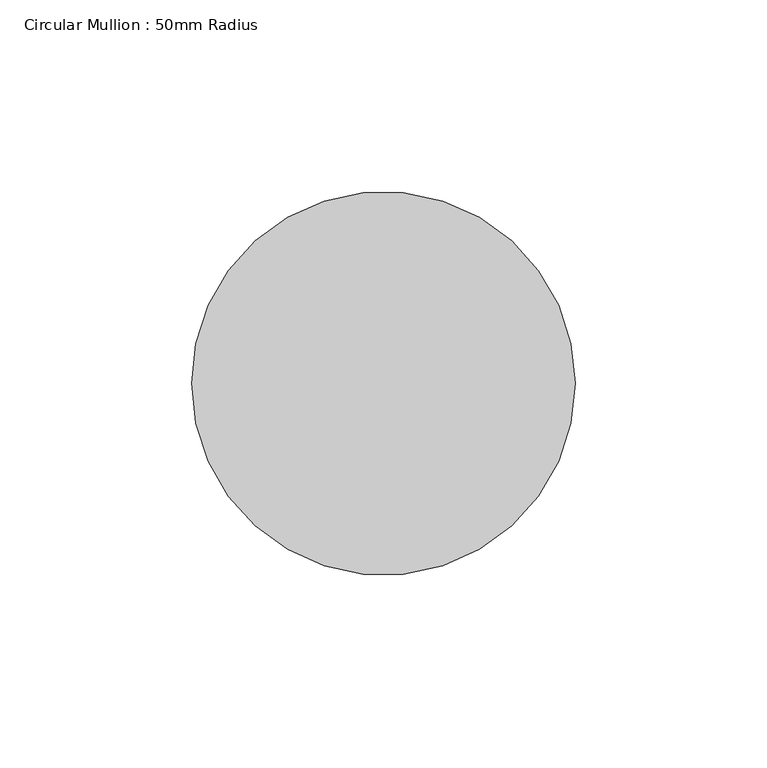
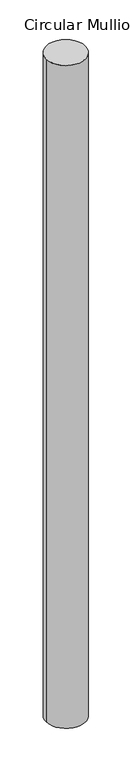
"""IFC4 building model written with IfcOpenShell, lengths in millimetres: member geometry, Circular Mullion : 50mm Radius."""

import ifcopenshell
import ifcopenshell.guid

model = None  # the IFC model being written
_history = None  # IfcOwnerHistory: only IFC2X3 demands one
_inside = {}  # id of a spatial element -> (the spatial element, [elements in it])
_under = {}  # id of a project, library or spatial element -> (it, [spatial elements below it])
_declared = {}  # id of a project -> (the project, [libraries it declares])
_typed = {}  # id of a type object -> (the type object, [elements of that type])
_made_of = {}  # id of a material, layer set ... -> (it, [elements and type objects made of it])


def new_model(schema):
    """Start an empty IFC model of exactly this schema.

    Asked for "IFC4X3", IfcOpenShell would pick the latest addendum, in which some entities
    have other attributes; the version numbers below select the first issue.
    IFC2X3 requires an IfcOwnerHistory on every rooted entity: one is made here for all.
    """
    global model, _history
    if schema == "IFC4X3":
        model = ifcopenshell.file(schema_version=(4, 3, 0, 0))
    else:
        model = ifcopenshell.file(schema=schema)
    _inside.clear()
    _under.clear()
    _declared.clear()
    _typed.clear()
    _made_of.clear()
    _history = None
    if model.schema == "IFC2X3":
        org = make("IfcOrganization", Name="unknown")
        user = make(
            "IfcPersonAndOrganization",
            ThePerson=make("IfcPerson", FamilyName="unknown"),
            TheOrganization=org,
        )
        app = make(
            "IfcApplication",
            ApplicationDeveloper=org,
            Version="unknown",
            ApplicationFullName="unknown",
            ApplicationIdentifier="unknown",
        )
        _history = make(
            "IfcOwnerHistory",
            OwningUser=user,
            OwningApplication=app,
            ChangeAction="ADDED",
            CreationDate=0,
        )
    return model


def make(cls, **values):
    """One entity of the class cls with the attributes given. An attribute that is None is left unset."""
    return model.create_entity(
        cls, **{name: value for name, value in values.items() if value is not None}
    )


def rooted(cls, **values):
    """An entity with a GlobalId (a new one), such as an element, a storey or a relation."""
    return make(cls, GlobalId=ifcopenshell.guid.new(), OwnerHistory=_history, **values)


def si_unit(unit_type, name, prefix=None):
    """IfcSIUnit, for example si_unit("LENGTHUNIT", "METRE", prefix="MILLI")."""
    return make("IfcSIUnit", UnitType=unit_type, Prefix=prefix, Name=name)


def assignment(units):
    """IfcUnitAssignment: the units of a project."""
    return None if units is None else make("IfcUnitAssignment", Units=units)


def point(xyz):
    """IfcCartesianPoint."""
    return None if xyz is None else make("IfcCartesianPoint", Coordinates=xyz)


def direction(xyz):
    """IfcDirection."""
    return None if xyz is None else make("IfcDirection", DirectionRatios=xyz)


def frame(location, z_axis=None, x_axis=None):
    """IfcAxis2Placement3D, a coordinate frame: its origin and axes. An axis left out is left unset."""
    return make(
        "IfcAxis2Placement3D",
        Location=point(location),
        Axis=direction(z_axis),
        RefDirection=direction(x_axis),
    )


def frame_2d(location, x_axis=None):
    """IfcAxis2Placement2D, a coordinate frame in the plane: its origin and x axis."""
    return make(
        "IfcAxis2Placement2D", Location=point(location), RefDirection=direction(x_axis)
    )


def origin():
    """The frame at (0, 0, 0) with its axes left unset."""
    return frame((0.0, 0.0, 0.0))


def origin_2d():
    """The frame at (0, 0) in the plane with its x axis left unset."""
    return frame_2d((0.0, 0.0))


def place(relative_to, where):
    """IfcLocalPlacement: puts the frame where relative to a parent placement (None: the world)."""
    return make(
        "IfcLocalPlacement", PlacementRelTo=relative_to, RelativePlacement=where
    )


def context(
    kind, dimensions, precision=None, world=None, true_north=None, identifier=None
):
    """IfcGeometricRepresentationContext, for example the 3D "Model" context."""
    return make(
        "IfcGeometricRepresentationContext",
        ContextIdentifier=identifier,
        ContextType=kind,
        CoordinateSpaceDimension=dimensions,
        Precision=precision,
        WorldCoordinateSystem=world,
        TrueNorth=true_north,
    )


def project(units=None, contexts=None):
    """IfcProject with its units and contexts."""
    return rooted(
        "IfcProject",
        Name="project",
        RepresentationContexts=contexts,
        UnitsInContext=assignment(units),
    )


def spatial(cls, under=None, at=None, **own):
    """A site, building, storey or space (cls), placed at a placement, below another one or the project."""
    s = rooted(cls, ObjectPlacement=at, **own)
    if under is not None:
        _under.setdefault(under.id(), (under, []))[1].append(s)
    return s


def circle_curve(where, radius):
    """IfcCircle in the frame where."""
    return make("IfcCircle", Position=where, Radius=radius)


def trimmed(basis, trim1, trim2, sense, master):
    """IfcTrimmedCurve: the piece of a basis curve between two trims."""
    return make(
        "IfcTrimmedCurve",
        BasisCurve=basis,
        Trim1=trim1,
        Trim2=trim2,
        SenseAgreement=sense,
        MasterRepresentation=master,
    )


def segment(curve, same_sense, transition):
    """IfcCompositeCurveSegment."""
    return make(
        "IfcCompositeCurveSegment",
        Transition=transition,
        SameSense=same_sense,
        ParentCurve=curve,
    )


def composite_curve(segments, self_intersect=None):
    """IfcCompositeCurve: segments joined end to end."""
    return make("IfcCompositeCurve", Segments=segments, SelfIntersect=self_intersect)


def outline(outer, holes=None, kind="AREA"):
    """IfcArbitraryClosedProfileDef: a profile drawn as a closed curve; with holes, ...WithVoids."""
    if holes is None:
        return make("IfcArbitraryClosedProfileDef", ProfileType=kind, OuterCurve=outer)
    return make(
        "IfcArbitraryProfileDefWithVoids",
        ProfileType=kind,
        OuterCurve=outer,
        InnerCurves=holes,
    )


def extrude(swept, where, along, depth):
    """IfcExtrudedAreaSolid: the profile swept, set in the frame where, extruded along a direction by depth."""
    return make(
        "IfcExtrudedAreaSolid",
        SweptArea=swept,
        Position=where,
        ExtrudedDirection=direction(along),
        Depth=depth,
    )


def shape(context_of_items, identifier, shape_type, items):
    """IfcShapeRepresentation: the items that make up one representation, for example the "Body"."""
    return make(
        "IfcShapeRepresentation",
        ContextOfItems=context_of_items,
        RepresentationIdentifier=identifier,
        RepresentationType=shape_type,
        Items=items,
    )


def source(mapping_origin, context_of_items, identifier, shape_type, items):
    """IfcRepresentationMap: a shape defined once, which mapped items show again and again."""
    return make(
        "IfcRepresentationMap",
        MappingOrigin=mapping_origin,
        MappedRepresentation=shape(context_of_items, identifier, shape_type, items),
    )


def transform(
    local_origin,
    x_axis=None,
    y_axis=None,
    z_axis=None,
    scale=None,
    scale2=None,
    scale3=None,
    uniform=True,
):
    """IfcCartesianTransformationOperator3D, or its non-uniform kind. x_axis, y_axis, z_axis: its Axis1, 2, 3."""
    if uniform:
        return make(
            "IfcCartesianTransformationOperator3D",
            Axis1=direction(x_axis),
            Axis2=direction(y_axis),
            LocalOrigin=point(local_origin),
            Scale=scale,
            Axis3=direction(z_axis),
        )
    return make(
        "IfcCartesianTransformationOperator3DnonUniform",
        Axis1=direction(x_axis),
        Axis2=direction(y_axis),
        LocalOrigin=point(local_origin),
        Scale=scale,
        Axis3=direction(z_axis),
        Scale2=scale2,
        Scale3=scale3,
    )


def mapped(mapping_source, mapping_target):
    """IfcMappedItem: shows the shape of a source again, moved by a transform."""
    return make(
        "IfcMappedItem", MappingSource=mapping_source, MappingTarget=mapping_target
    )


def made_of(thing, what):
    """Note that an element or type object is made of a material, layer set ...; save() writes the relation."""
    if what is not None:
        _made_of.setdefault(what.id(), (what, []))[1].append(thing)
    return thing


def element(
    cls,
    number,
    at=None,
    inside=None,
    cuts=None,
    type_object=None,
    material=None,
    context=None,
    identifier="Body",
    shape_type=None,
    held_by="IfcProductDefinitionShape",
    body=None,
    shapes=None,
    **own,
):
    """One element of the class cls, such as IfcWall. Its Tag is "e" and its number.

    at: its placement. inside: the storey or other place that contains it. cuts: it is an
    opening in that element (IfcRelVoidsElement). A single representation is given by context,
    identifier, shape_type and body (its items); several are given by shapes. held_by: the class
    of the entity that holds the representations. save() writes the other relations.
    """
    e = rooted(cls, Tag="e%d" % number, ObjectPlacement=at, **own)
    if body is not None:
        shapes = [shape(context, identifier, shape_type, body)]
    if shapes is not None:
        e.Representation = make(held_by, Representations=shapes)
    if inside is not None:
        _inside.setdefault(inside.id(), (inside, []))[1].append(e)
    if cuts is not None:
        rooted(
            "IfcRelVoidsElement", RelatingBuildingElement=cuts, RelatedOpeningElement=e
        )
    if type_object is not None:
        _typed.setdefault(type_object.id(), (type_object, []))[1].append(e)
    return made_of(e, material)


def aggregate(whole, parts):
    """IfcRelAggregates: a whole, such as a stair, and the parts it consists of."""
    return rooted("IfcRelAggregates", RelatingObject=whole, RelatedObjects=parts)


def save(model, path):
    """Write the relations noted so far, then the file.

    IfcRelAggregates (storeys below a building ...), IfcRelContainedInSpatialStructure (elements
    in a storey), IfcRelDefinesByType, IfcRelAssociatesMaterial and IfcRelDeclares: one each for
    every whole, place, type object, material and project.
    """
    for whole, parts in _under.values():
        aggregate(whole, parts)
    for where, things in _inside.values():
        rooted(
            "IfcRelContainedInSpatialStructure",
            RelatedElements=things,
            RelatingStructure=where,
        )
    for kind, things in _typed.values():
        rooted("IfcRelDefinesByType", RelatedObjects=things, RelatingType=kind)
    for what, things in _made_of.values():
        rooted("IfcRelAssociatesMaterial", RelatedObjects=things, RelatingMaterial=what)
    for by, libraries in _declared.values():
        rooted("IfcRelDeclares", RelatingContext=by, RelatedDefinitions=libraries)
    model.write(path)


def circular_mullion_50mm_radius_0641689d(model_context):
    return source(origin(), model_context, "Body", "SweptSolid", [
        extrude(outline(composite_curve([segment(trimmed(circle_curve(origin_2d(), 50.0), [point((50.0, 0.0))], [point((-50.0, 0.0))], False, "CARTESIAN"), True, "CONTINUOUS"), segment(trimmed(circle_curve(origin_2d(), 50.0), [point((-50.0, 0.0))], [point((50.0, 0.0))], False, "CARTESIAN"), True, "CONTINUOUS")], self_intersect=False)), frame((0.0, 0.0, -1791.6410056), z_axis=(0.0, 0.0, 1.0), x_axis=(1.0, 0.0, 0.0)), (0.0, 0.0, 1.0), 1791.6410056),
    ])


if __name__ == "__main__":
    model = new_model("IFC4")
    model_context = context("Model", 3, world=origin())
    ifc_project = project(units=[si_unit("LENGTHUNIT", "METRE", prefix="MILLI")], contexts=[model_context])
    site = spatial("IfcSite", under=ifc_project)
    building = spatial("IfcBuilding", under=site)
    placement = place(None, origin())
    circular_mullion_50mm_radius_shape = circular_mullion_50mm_radius_0641689d(model_context)
    element("IfcMember", 1, ObjectType="Circular Mullion : 50mm Radius", at=placement, inside=building, context=model_context, shape_type="MappedRepresentation", body=[
        mapped(circular_mullion_50mm_radius_shape, transform((0.0, 0.0, 0.0), x_axis=(1.0, 0.0, 0.0), y_axis=(0.0, 1.0, 0.0), z_axis=(0.0, 0.0, 1.0))),
    ])
    save(model, "model.ifc")

# Revit data of these elements
# Type "Circular Mullion : 50mm Radius"
#   built-in parameter 1007350 = 0.164042 (stored number, unit not read)
# Element 1 (IfcMember, "Circular Mullion : 50mm Radius")
#   Materials on its faces: "Aluminium"
# Materials
#   "Aluminium": class "Metal", colour RGB 247 247 247, transparency 0, Description = "Aluminium 6061", Cost = 0
